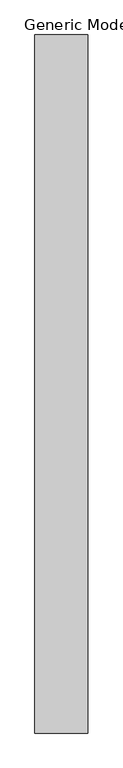
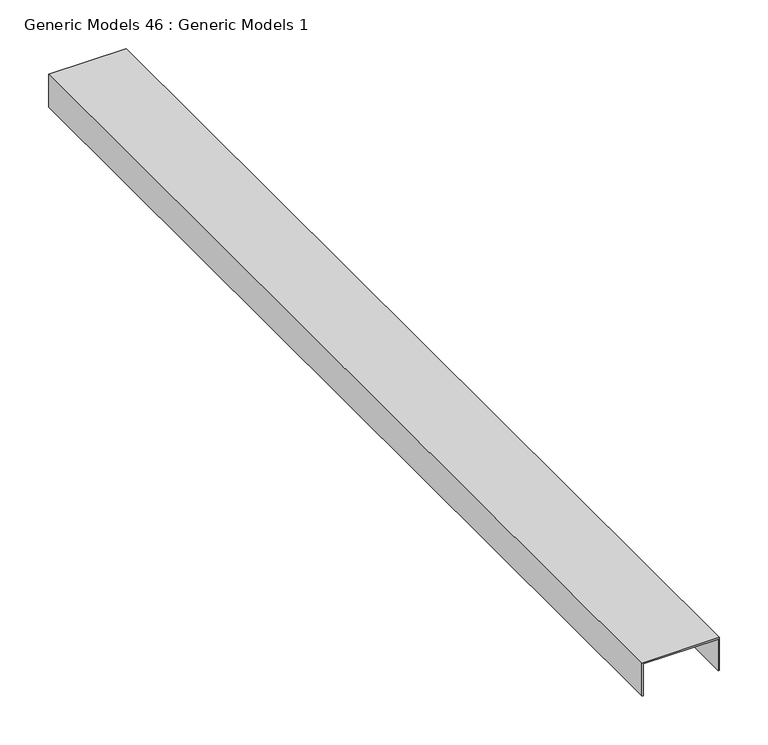
"""IFC4 building model written with IfcOpenShell, lengths in millimetres: proxy geometry, Generic Models 46 : Generic Models 1."""

import ifcopenshell
import ifcopenshell.guid

model = None  # the IFC model being written
_history = None  # IfcOwnerHistory: only IFC2X3 demands one
_inside = {}  # id of a spatial element -> (the spatial element, [elements in it])
_under = {}  # id of a project, library or spatial element -> (it, [spatial elements below it])
_declared = {}  # id of a project -> (the project, [libraries it declares])
_typed = {}  # id of a type object -> (the type object, [elements of that type])
_made_of = {}  # id of a material, layer set ... -> (it, [elements and type objects made of it])


def new_model(schema):
    """Start an empty IFC model of exactly this schema.

    Asked for "IFC4X3", IfcOpenShell would pick the latest addendum, in which some entities
    have other attributes; the version numbers below select the first issue.
    IFC2X3 requires an IfcOwnerHistory on every rooted entity: one is made here for all.
    """
    global model, _history
    if schema == "IFC4X3":
        model = ifcopenshell.file(schema_version=(4, 3, 0, 0))
    else:
        model = ifcopenshell.file(schema=schema)
    _inside.clear()
    _under.clear()
    _declared.clear()
    _typed.clear()
    _made_of.clear()
    _history = None
    if model.schema == "IFC2X3":
        org = make("IfcOrganization", Name="unknown")
        user = make(
            "IfcPersonAndOrganization",
            ThePerson=make("IfcPerson", FamilyName="unknown"),
            TheOrganization=org,
        )
        app = make(
            "IfcApplication",
            ApplicationDeveloper=org,
            Version="unknown",
            ApplicationFullName="unknown",
            ApplicationIdentifier="unknown",
        )
        _history = make(
            "IfcOwnerHistory",
            OwningUser=user,
            OwningApplication=app,
            ChangeAction="ADDED",
            CreationDate=0,
        )
    return model


def make(cls, **values):
    """One entity of the class cls with the attributes given. An attribute that is None is left unset."""
    return model.create_entity(
        cls, **{name: value for name, value in values.items() if value is not None}
    )


def rooted(cls, **values):
    """An entity with a GlobalId (a new one), such as an element, a storey or a relation."""
    return make(cls, GlobalId=ifcopenshell.guid.new(), OwnerHistory=_history, **values)


def si_unit(unit_type, name, prefix=None):
    """IfcSIUnit, for example si_unit("LENGTHUNIT", "METRE", prefix="MILLI")."""
    return make("IfcSIUnit", UnitType=unit_type, Prefix=prefix, Name=name)


def assignment(units):
    """IfcUnitAssignment: the units of a project."""
    return None if units is None else make("IfcUnitAssignment", Units=units)


def point(xyz):
    """IfcCartesianPoint."""
    return None if xyz is None else make("IfcCartesianPoint", Coordinates=xyz)


def direction(xyz):
    """IfcDirection."""
    return None if xyz is None else make("IfcDirection", DirectionRatios=xyz)


def frame(location, z_axis=None, x_axis=None):
    """IfcAxis2Placement3D, a coordinate frame: its origin and axes. An axis left out is left unset."""
    return make(
        "IfcAxis2Placement3D",
        Location=point(location),
        Axis=direction(z_axis),
        RefDirection=direction(x_axis),
    )


def origin():
    """The frame at (0, 0, 0) with its axes left unset."""
    return frame((0.0, 0.0, 0.0))


def place(relative_to, where):
    """IfcLocalPlacement: puts the frame where relative to a parent placement (None: the world)."""
    return make(
        "IfcLocalPlacement", PlacementRelTo=relative_to, RelativePlacement=where
    )


def context(
    kind, dimensions, precision=None, world=None, true_north=None, identifier=None
):
    """IfcGeometricRepresentationContext, for example the 3D "Model" context."""
    return make(
        "IfcGeometricRepresentationContext",
        ContextIdentifier=identifier,
        ContextType=kind,
        CoordinateSpaceDimension=dimensions,
        Precision=precision,
        WorldCoordinateSystem=world,
        TrueNorth=true_north,
    )


def project(units=None, contexts=None):
    """IfcProject with its units and contexts."""
    return rooted(
        "IfcProject",
        Name="project",
        RepresentationContexts=contexts,
        UnitsInContext=assignment(units),
    )


def spatial(cls, under=None, at=None, **own):
    """A site, building, storey or space (cls), placed at a placement, below another one or the project."""
    s = rooted(cls, ObjectPlacement=at, **own)
    if under is not None:
        _under.setdefault(under.id(), (under, []))[1].append(s)
    return s


def polyline(points):
    """IfcPolyline through the points."""
    return make("IfcPolyline", Points=[point(p) for p in points])


def outline(outer, holes=None, kind="AREA"):
    """IfcArbitraryClosedProfileDef: a profile drawn as a closed curve; with holes, ...WithVoids."""
    if holes is None:
        return make("IfcArbitraryClosedProfileDef", ProfileType=kind, OuterCurve=outer)
    return make(
        "IfcArbitraryProfileDefWithVoids",
        ProfileType=kind,
        OuterCurve=outer,
        InnerCurves=holes,
    )


def extrude(swept, where, along, depth):
    """IfcExtrudedAreaSolid: the profile swept, set in the frame where, extruded along a direction by depth."""
    return make(
        "IfcExtrudedAreaSolid",
        SweptArea=swept,
        Position=where,
        ExtrudedDirection=direction(along),
        Depth=depth,
    )


def shape(context_of_items, identifier, shape_type, items):
    """IfcShapeRepresentation: the items that make up one representation, for example the "Body"."""
    return make(
        "IfcShapeRepresentation",
        ContextOfItems=context_of_items,
        RepresentationIdentifier=identifier,
        RepresentationType=shape_type,
        Items=items,
    )


def source(mapping_origin, context_of_items, identifier, shape_type, items):
    """IfcRepresentationMap: a shape defined once, which mapped items show again and again."""
    return make(
        "IfcRepresentationMap",
        MappingOrigin=mapping_origin,
        MappedRepresentation=shape(context_of_items, identifier, shape_type, items),
    )


def transform(
    local_origin,
    x_axis=None,
    y_axis=None,
    z_axis=None,
    scale=None,
    scale2=None,
    scale3=None,
    uniform=True,
):
    """IfcCartesianTransformationOperator3D, or its non-uniform kind. x_axis, y_axis, z_axis: its Axis1, 2, 3."""
    if uniform:
        return make(
            "IfcCartesianTransformationOperator3D",
            Axis1=direction(x_axis),
            Axis2=direction(y_axis),
            LocalOrigin=point(local_origin),
            Scale=scale,
            Axis3=direction(z_axis),
        )
    return make(
        "IfcCartesianTransformationOperator3DnonUniform",
        Axis1=direction(x_axis),
        Axis2=direction(y_axis),
        LocalOrigin=point(local_origin),
        Scale=scale,
        Axis3=direction(z_axis),
        Scale2=scale2,
        Scale3=scale3,
    )


def mapped(mapping_source, mapping_target):
    """IfcMappedItem: shows the shape of a source again, moved by a transform."""
    return make(
        "IfcMappedItem", MappingSource=mapping_source, MappingTarget=mapping_target
    )


def made_of(thing, what):
    """Note that an element or type object is made of a material, layer set ...; save() writes the relation."""
    if what is not None:
        _made_of.setdefault(what.id(), (what, []))[1].append(thing)
    return thing


def element(
    cls,
    number,
    at=None,
    inside=None,
    cuts=None,
    type_object=None,
    material=None,
    context=None,
    identifier="Body",
    shape_type=None,
    held_by="IfcProductDefinitionShape",
    body=None,
    shapes=None,
    **own,
):
    """One element of the class cls, such as IfcWall. Its Tag is "e" and its number.

    at: its placement. inside: the storey or other place that contains it. cuts: it is an
    opening in that element (IfcRelVoidsElement). A single representation is given by context,
    identifier, shape_type and body (its items); several are given by shapes. held_by: the class
    of the entity that holds the representations. save() writes the other relations.
    """
    e = rooted(cls, Tag="e%d" % number, ObjectPlacement=at, **own)
    if body is not None:
        shapes = [shape(context, identifier, shape_type, body)]
    if shapes is not None:
        e.Representation = make(held_by, Representations=shapes)
    if inside is not None:
        _inside.setdefault(inside.id(), (inside, []))[1].append(e)
    if cuts is not None:
        rooted(
            "IfcRelVoidsElement", RelatingBuildingElement=cuts, RelatedOpeningElement=e
        )
    if type_object is not None:
        _typed.setdefault(type_object.id(), (type_object, []))[1].append(e)
    return made_of(e, material)


def aggregate(whole, parts):
    """IfcRelAggregates: a whole, such as a stair, and the parts it consists of."""
    return rooted("IfcRelAggregates", RelatingObject=whole, RelatedObjects=parts)


def save(model, path):
    """Write the relations noted so far, then the file.

    IfcRelAggregates (storeys below a building ...), IfcRelContainedInSpatialStructure (elements
    in a storey), IfcRelDefinesByType, IfcRelAssociatesMaterial and IfcRelDeclares: one each for
    every whole, place, type object, material and project.
    """
    for whole, parts in _under.values():
        aggregate(whole, parts)
    for where, things in _inside.values():
        rooted(
            "IfcRelContainedInSpatialStructure",
            RelatedElements=things,
            RelatingStructure=where,
        )
    for kind, things in _typed.values():
        rooted("IfcRelDefinesByType", RelatedObjects=things, RelatingType=kind)
    for what, things in _made_of.values():
        rooted("IfcRelAssociatesMaterial", RelatedObjects=things, RelatingMaterial=what)
    for by, libraries in _declared.values():
        rooted("IfcRelDeclares", RelatingContext=by, RelatedDefinitions=libraries)
    model.write(path)


def generic_models_46_generic_models_1_467ce512(model_context):
    return source(origin(), model_context, "Body", "SweptSolid", [
        extrude(outline(polyline([(393.2679367, 50793.65), (351.9929367, 50793.65), (351.9929367, 50795.2375), (391.6804367, 50795.2375), (391.6804367, 50884.1375), (351.9929367, 50884.1375), (351.9929367, 50885.725), (393.2679367, 50885.725), (393.2679367, 50793.65)])), frame((0.0, 0.0, 0.0), z_axis=(0.0, 1.0, 0.0), x_axis=(0.0, 0.0, 1.0)), (0.0, 0.0, 1.0), 1219.2),
    ])


if __name__ == "__main__":
    model = new_model("IFC4")
    model_context = context("Model", 3, world=origin())
    ifc_project = project(units=[si_unit("LENGTHUNIT", "METRE", prefix="MILLI")], contexts=[model_context])
    site = spatial("IfcSite", under=ifc_project)
    building = spatial("IfcBuilding", under=site)
    placement = place(None, origin())
    generic_models_46_generic_models_1_shape = generic_models_46_generic_models_1_467ce512(model_context)
    element("IfcBuildingElementProxy", 1, Name="Generic Models 46 : Generic Models 1", ObjectType="Generic Models 46 : Generic Models 1", at=placement, inside=building, context=model_context, shape_type="MappedRepresentation", body=[
        mapped(generic_models_46_generic_models_1_shape, transform((0.0, 0.0, 0.0), x_axis=(1.0, 0.0, 0.0), y_axis=(0.0, 1.0, 0.0), z_axis=(0.0, 0.0, 1.0))),
    ])
    save(model, "model.ifc")

# Revit data of these elements
# Element 1 (IfcBuildingElementProxy, "Generic Models 46 : Generic Models 1")
#   Materials on its faces: "METAL RUNNER ANCHORED TO STRUCTURE"
# Materials
#   "METAL RUNNER ANCHORED TO STRUCTURE": class "Unassigned", colour RGB 210 209 208, transparency 0, Keynote = "M05121300.02", Cost = 0
